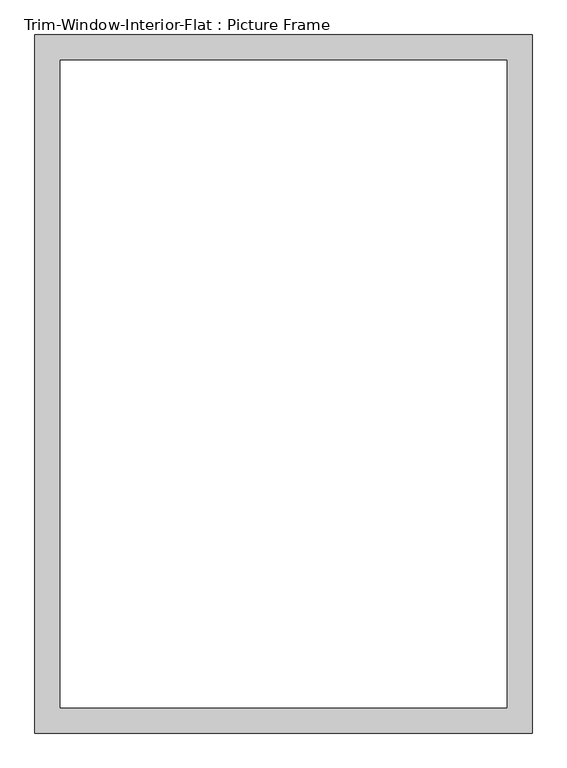
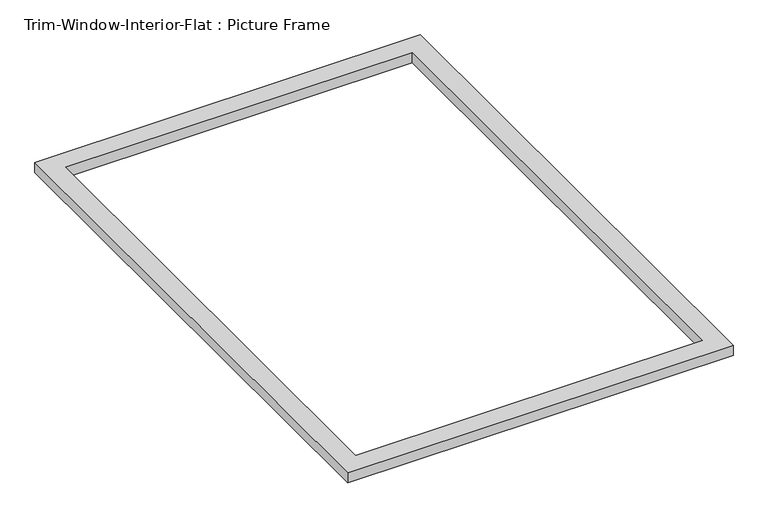
"""IFC4 building model written with IfcOpenShell, lengths in millimetres: proxy geometry, Trim-Window-Interior-Flat : Picture Frame."""

from ifc_helpers import new_model, si_unit, origin, origin_with_axes, place, context, project, spatial, polyline, outline, extrude, source, transform, mapped, element, save


def trim_window_interior_flat_picture_frame_82b38731(model_context):
    return source(origin(), model_context, "Body", "SweptSolid", [
        extrude(outline(polyline([(565.15, -44.45), (-565.15, -44.45), (-565.15, 1543.05), (565.15, 1543.05), (565.15, -44.45)]), holes=[polyline([(508.0, 12.7), (508.0, 1485.9), (-508.0, 1485.9), (-508.0, 12.7), (508.0, 12.7)])]), origin_with_axes(), (0.0, 0.0, 1.0), 31.75),
    ])


if __name__ == "__main__":
    model = new_model("IFC4")
    model_context = context("Model", 3, world=origin())
    ifc_project = project(units=[si_unit("LENGTHUNIT", "METRE", prefix="MILLI")], contexts=[model_context])
    site = spatial("IfcSite", under=ifc_project)
    building = spatial("IfcBuilding", under=site)
    placement = place(None, origin())
    trim_window_interior_flat_picture_frame_shape = trim_window_interior_flat_picture_frame_82b38731(model_context)
    element("IfcBuildingElementProxy", 1, Name="Trim-Window-Interior-Flat : Picture Frame", ObjectType="Trim-Window-Interior-Flat : Picture Frame", at=placement, inside=building, context=model_context, shape_type="MappedRepresentation", body=[
        mapped(trim_window_interior_flat_picture_frame_shape, transform((0.0, 0.0, 0.0), x_axis=(1.0, 0.0, 0.0), y_axis=(0.0, 1.0, 0.0), z_axis=(0.0, 0.0, 1.0))),
    ])
    save(model, "model.ifc")

# Revit data of these elements
# Type "Trim-Window-Interior-Flat : Picture Frame"
#   Trim Thickness_Picture Frame = 0' - 1 1/4"
#   Trim Width = 0' - 2 1/4"
#   Trim Thickness_with Sill = 0' - 0 3/4"
#   Sill Thickness = 0' - 1 1/4"
#   Opening Width [instance default] = 2' - 0"
#   Opening Height [instance default] = 3' - 0"
#   Default Elevation = 4' - 0"
#   Sill = no
#   Picture Frame = yes
#   Trim Material [instance default] = none
# Element 1 (IfcBuildingElementProxy, "Trim-Window-Interior-Flat : Picture Frame")
#   Opening Width = 3' - 5"
#   Opening Height = 4' - 11"
#   Trim Material = Wood - Stained
#   Materials on its faces: "Wood - Stained"
# Materials
#   "Wood - Stained": class "Wood", colour RGB 224 178 126, transparency 0, Cost = 0
